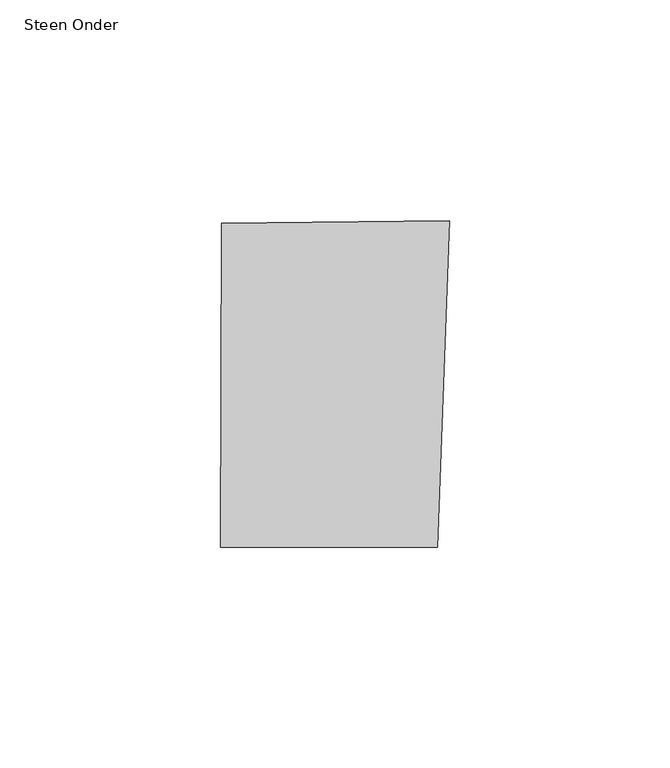
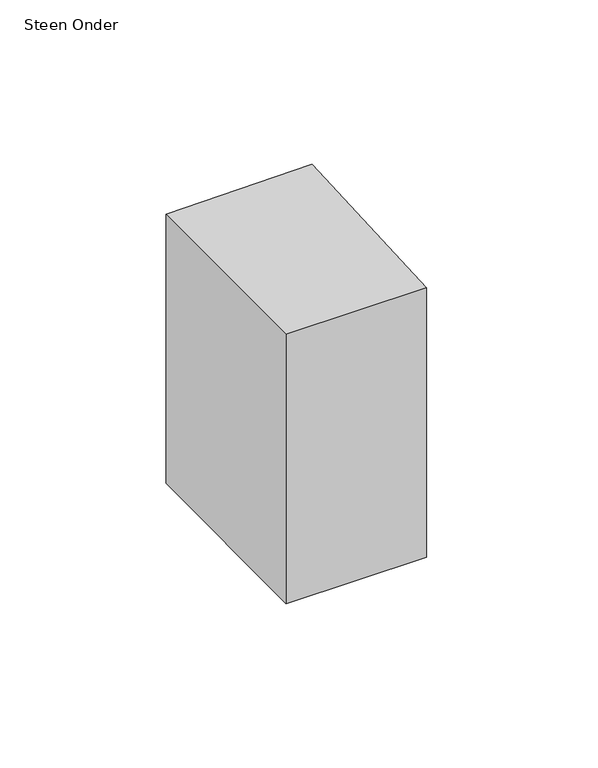
"""IFC4 building model written with IfcOpenShell, lengths in millimetres: proxy geometry, 00_GMA_steen_versie_4 : Steen Onder."""

import ifcopenshell
import ifcopenshell.guid

model = None  # the IFC model being written
_history = None  # IfcOwnerHistory: only IFC2X3 demands one
_inside = {}  # id of a spatial element -> (the spatial element, [elements in it])
_under = {}  # id of a project, library or spatial element -> (it, [spatial elements below it])
_declared = {}  # id of a project -> (the project, [libraries it declares])
_typed = {}  # id of a type object -> (the type object, [elements of that type])
_made_of = {}  # id of a material, layer set ... -> (it, [elements and type objects made of it])


def new_model(schema):
    """Start an empty IFC model of exactly this schema.

    Asked for "IFC4X3", IfcOpenShell would pick the latest addendum, in which some entities
    have other attributes; the version numbers below select the first issue.
    IFC2X3 requires an IfcOwnerHistory on every rooted entity: one is made here for all.
    """
    global model, _history
    if schema == "IFC4X3":
        model = ifcopenshell.file(schema_version=(4, 3, 0, 0))
    else:
        model = ifcopenshell.file(schema=schema)
    _inside.clear()
    _under.clear()
    _declared.clear()
    _typed.clear()
    _made_of.clear()
    _history = None
    if model.schema == "IFC2X3":
        org = make("IfcOrganization", Name="unknown")
        user = make(
            "IfcPersonAndOrganization",
            ThePerson=make("IfcPerson", FamilyName="unknown"),
            TheOrganization=org,
        )
        app = make(
            "IfcApplication",
            ApplicationDeveloper=org,
            Version="unknown",
            ApplicationFullName="unknown",
            ApplicationIdentifier="unknown",
        )
        _history = make(
            "IfcOwnerHistory",
            OwningUser=user,
            OwningApplication=app,
            ChangeAction="ADDED",
            CreationDate=0,
        )
    return model


def make(cls, **values):
    """One entity of the class cls with the attributes given. An attribute that is None is left unset."""
    return model.create_entity(
        cls, **{name: value for name, value in values.items() if value is not None}
    )


def rooted(cls, **values):
    """An entity with a GlobalId (a new one), such as an element, a storey or a relation."""
    return make(cls, GlobalId=ifcopenshell.guid.new(), OwnerHistory=_history, **values)


def si_unit(unit_type, name, prefix=None):
    """IfcSIUnit, for example si_unit("LENGTHUNIT", "METRE", prefix="MILLI")."""
    return make("IfcSIUnit", UnitType=unit_type, Prefix=prefix, Name=name)


def assignment(units):
    """IfcUnitAssignment: the units of a project."""
    return None if units is None else make("IfcUnitAssignment", Units=units)


def point(xyz):
    """IfcCartesianPoint."""
    return None if xyz is None else make("IfcCartesianPoint", Coordinates=xyz)


def direction(xyz):
    """IfcDirection."""
    return None if xyz is None else make("IfcDirection", DirectionRatios=xyz)


def frame(location, z_axis=None, x_axis=None):
    """IfcAxis2Placement3D, a coordinate frame: its origin and axes. An axis left out is left unset."""
    return make(
        "IfcAxis2Placement3D",
        Location=point(location),
        Axis=direction(z_axis),
        RefDirection=direction(x_axis),
    )


def origin():
    """The frame at (0, 0, 0) with its axes left unset."""
    return frame((0.0, 0.0, 0.0))


def origin_with_axes():
    """The frame at (0, 0, 0) with the z axis (0, 0, 1) and the x axis (1, 0, 0) written out."""
    return frame((0.0, 0.0, 0.0), z_axis=(0.0, 0.0, 1.0), x_axis=(1.0, 0.0, 0.0))


def place(relative_to, where):
    """IfcLocalPlacement: puts the frame where relative to a parent placement (None: the world)."""
    return make(
        "IfcLocalPlacement", PlacementRelTo=relative_to, RelativePlacement=where
    )


def context(
    kind, dimensions, precision=None, world=None, true_north=None, identifier=None
):
    """IfcGeometricRepresentationContext, for example the 3D "Model" context."""
    return make(
        "IfcGeometricRepresentationContext",
        ContextIdentifier=identifier,
        ContextType=kind,
        CoordinateSpaceDimension=dimensions,
        Precision=precision,
        WorldCoordinateSystem=world,
        TrueNorth=true_north,
    )


def project(units=None, contexts=None):
    """IfcProject with its units and contexts."""
    return rooted(
        "IfcProject",
        Name="project",
        RepresentationContexts=contexts,
        UnitsInContext=assignment(units),
    )


def spatial(cls, under=None, at=None, **own):
    """A site, building, storey or space (cls), placed at a placement, below another one or the project."""
    s = rooted(cls, ObjectPlacement=at, **own)
    if under is not None:
        _under.setdefault(under.id(), (under, []))[1].append(s)
    return s


def polyline(points):
    """IfcPolyline through the points."""
    return make("IfcPolyline", Points=[point(p) for p in points])


def outline(outer, holes=None, kind="AREA"):
    """IfcArbitraryClosedProfileDef: a profile drawn as a closed curve; with holes, ...WithVoids."""
    if holes is None:
        return make("IfcArbitraryClosedProfileDef", ProfileType=kind, OuterCurve=outer)
    return make(
        "IfcArbitraryProfileDefWithVoids",
        ProfileType=kind,
        OuterCurve=outer,
        InnerCurves=holes,
    )


def extrude(swept, where, along, depth):
    """IfcExtrudedAreaSolid: the profile swept, set in the frame where, extruded along a direction by depth."""
    return make(
        "IfcExtrudedAreaSolid",
        SweptArea=swept,
        Position=where,
        ExtrudedDirection=direction(along),
        Depth=depth,
    )


def shape(context_of_items, identifier, shape_type, items):
    """IfcShapeRepresentation: the items that make up one representation, for example the "Body"."""
    return make(
        "IfcShapeRepresentation",
        ContextOfItems=context_of_items,
        RepresentationIdentifier=identifier,
        RepresentationType=shape_type,
        Items=items,
    )


def source(mapping_origin, context_of_items, identifier, shape_type, items):
    """IfcRepresentationMap: a shape defined once, which mapped items show again and again."""
    return make(
        "IfcRepresentationMap",
        MappingOrigin=mapping_origin,
        MappedRepresentation=shape(context_of_items, identifier, shape_type, items),
    )


def transform(
    local_origin,
    x_axis=None,
    y_axis=None,
    z_axis=None,
    scale=None,
    scale2=None,
    scale3=None,
    uniform=True,
):
    """IfcCartesianTransformationOperator3D, or its non-uniform kind. x_axis, y_axis, z_axis: its Axis1, 2, 3."""
    if uniform:
        return make(
            "IfcCartesianTransformationOperator3D",
            Axis1=direction(x_axis),
            Axis2=direction(y_axis),
            LocalOrigin=point(local_origin),
            Scale=scale,
            Axis3=direction(z_axis),
        )
    return make(
        "IfcCartesianTransformationOperator3DnonUniform",
        Axis1=direction(x_axis),
        Axis2=direction(y_axis),
        LocalOrigin=point(local_origin),
        Scale=scale,
        Axis3=direction(z_axis),
        Scale2=scale2,
        Scale3=scale3,
    )


def mapped(mapping_source, mapping_target):
    """IfcMappedItem: shows the shape of a source again, moved by a transform."""
    return make(
        "IfcMappedItem", MappingSource=mapping_source, MappingTarget=mapping_target
    )


def made_of(thing, what):
    """Note that an element or type object is made of a material, layer set ...; save() writes the relation."""
    if what is not None:
        _made_of.setdefault(what.id(), (what, []))[1].append(thing)
    return thing


def element(
    cls,
    number,
    at=None,
    inside=None,
    cuts=None,
    type_object=None,
    material=None,
    context=None,
    identifier="Body",
    shape_type=None,
    held_by="IfcProductDefinitionShape",
    body=None,
    shapes=None,
    **own,
):
    """One element of the class cls, such as IfcWall. Its Tag is "e" and its number.

    at: its placement. inside: the storey or other place that contains it. cuts: it is an
    opening in that element (IfcRelVoidsElement). A single representation is given by context,
    identifier, shape_type and body (its items); several are given by shapes. held_by: the class
    of the entity that holds the representations. save() writes the other relations.
    """
    e = rooted(cls, Tag="e%d" % number, ObjectPlacement=at, **own)
    if body is not None:
        shapes = [shape(context, identifier, shape_type, body)]
    if shapes is not None:
        e.Representation = make(held_by, Representations=shapes)
    if inside is not None:
        _inside.setdefault(inside.id(), (inside, []))[1].append(e)
    if cuts is not None:
        rooted(
            "IfcRelVoidsElement", RelatingBuildingElement=cuts, RelatedOpeningElement=e
        )
    if type_object is not None:
        _typed.setdefault(type_object.id(), (type_object, []))[1].append(e)
    return made_of(e, material)


def aggregate(whole, parts):
    """IfcRelAggregates: a whole, such as a stair, and the parts it consists of."""
    return rooted("IfcRelAggregates", RelatingObject=whole, RelatedObjects=parts)


def save(model, path):
    """Write the relations noted so far, then the file.

    IfcRelAggregates (storeys below a building ...), IfcRelContainedInSpatialStructure (elements
    in a storey), IfcRelDefinesByType, IfcRelAssociatesMaterial and IfcRelDeclares: one each for
    every whole, place, type object, material and project.
    """
    for whole, parts in _under.values():
        aggregate(whole, parts)
    for where, things in _inside.values():
        rooted(
            "IfcRelContainedInSpatialStructure",
            RelatedElements=things,
            RelatingStructure=where,
        )
    for kind, things in _typed.values():
        rooted("IfcRelDefinesByType", RelatedObjects=things, RelatingType=kind)
    for what, things in _made_of.values():
        rooted("IfcRelAssociatesMaterial", RelatedObjects=things, RelatingMaterial=what)
    for by, libraries in _declared.values():
        rooted("IfcRelDeclares", RelatingContext=by, RelatedDefinitions=libraries)
    model.write(path)


def steen_onder_560c44af(model_context):
    return source(origin(), model_context, "Body", "SweptSolid", [
        extrude(outline(polyline([(101.7974389, 103.2596899), (99.1314471, 29.1297979), (49.8374632, 29.1379061), (50.0968702, 102.5898261), (101.7974389, 103.2596899)])), origin_with_axes(), (0.0, 0.0, 1.0), 100.0),
    ])


if __name__ == "__main__":
    model = new_model("IFC4")
    model_context = context("Model", 3, world=origin())
    ifc_project = project(units=[si_unit("LENGTHUNIT", "METRE", prefix="MILLI")], contexts=[model_context])
    site = spatial("IfcSite", under=ifc_project)
    building = spatial("IfcBuilding", under=site)
    placement = place(None, origin())
    steen_onder_shape = steen_onder_560c44af(model_context)
    element("IfcBuildingElementProxy", 1, Name="00_GMA_steen_versie_4 : Steen Onder", ObjectType="00_GMA_steen_versie_4 : Steen Onder", at=placement, inside=building, context=model_context, shape_type="MappedRepresentation", body=[
        mapped(steen_onder_shape, transform((0.0, 0.0, 0.0), x_axis=(1.0, 0.0, 0.0), y_axis=(0.0, 1.0, 0.0), z_axis=(0.0, 0.0, 1.0))),
    ])
    save(model, "model.ifc")

# Revit data of these elements
# Type "00_GMA_steen_versie_4 : Steen Onder"
#   StootVoegHalfBoven [instance default] = 5 mm
#   StootVoegHalf [instance default] = 5 mm
#   StootVoegBreedteOnder = 10 mm
#   StootVoegBreedteBoven = 10 mm
#   Steendikte = 100 mm
#   LintVoegOnderHalf = 0 mm
#   LintVoegOnder = 0 mm
#   LintVoegBovenHalf = 5 mm
#   LintVoegBoven = 10 mm
#   materiaal = none
#   MateriaalVoeg = none
#   Default Elevation = 0
